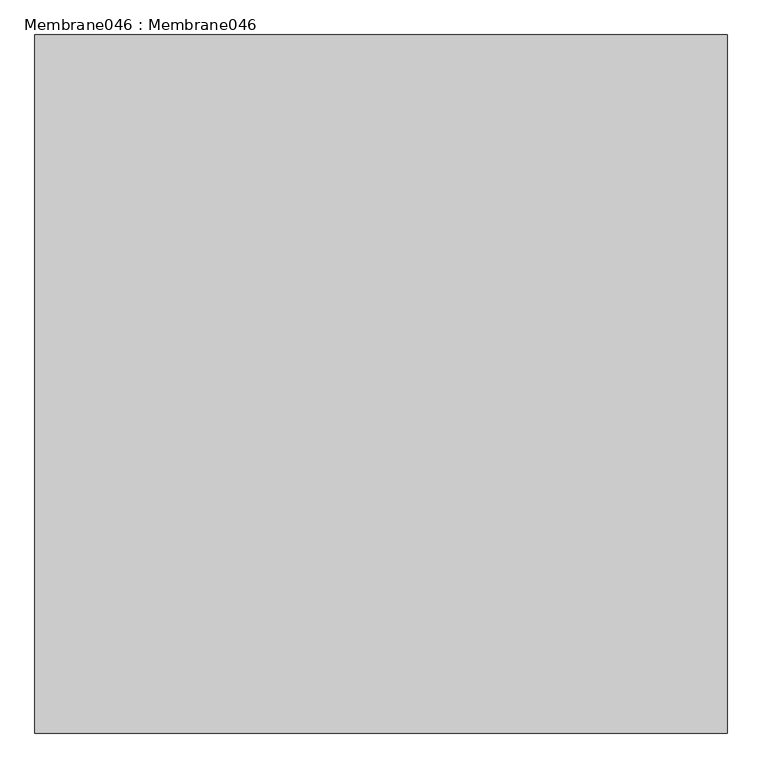
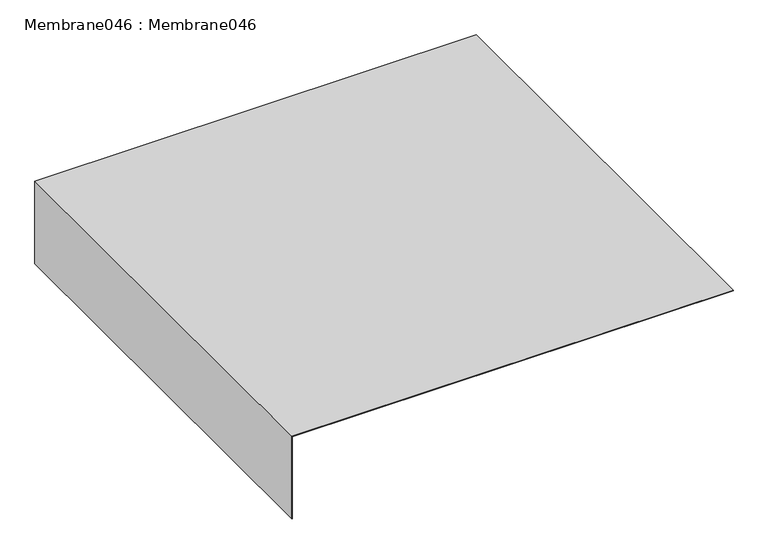
"""IFC4 building model written with IfcOpenShell, lengths in millimetres: proxy geometry, Membrane046 : Membrane046."""

from ifc_helpers import new_model, si_unit, frame, origin, place, context, project, spatial, polyline, outline, extrude, source, transform, mapped, element, save


def membrane046_membrane046_453448af(model_context):
    return source(origin(), model_context, "Body", "SweptSolid", [
        extrude(outline(polyline([(42521.46875, -475.8491821), (42521.46875, -2458.5124512), (42129.1953125, -2458.5124512), (42129.1953125, -2456.5124512), (42519.46875, -2456.5124512), (42519.46875, -475.8491821), (42521.46875, -475.8491821)])), frame((0.0, -1052.8906574, 0.0), z_axis=(0.0, 1.0, 0.0), x_axis=(0.0, 0.0, 1.0)), (0.0, 0.0, 1.0), 2000.0),
    ])


if __name__ == "__main__":
    model = new_model("IFC4")
    model_context = context("Model", 3, world=origin())
    ifc_project = project(units=[si_unit("LENGTHUNIT", "METRE", prefix="MILLI")], contexts=[model_context])
    site = spatial("IfcSite", under=ifc_project)
    building = spatial("IfcBuilding", under=site)
    placement = place(None, origin())
    membrane046_membrane046_shape = membrane046_membrane046_453448af(model_context)
    element("IfcBuildingElementProxy", 1, Name="Membrane046 : Membrane046", ObjectType="Membrane046 : Membrane046", at=placement, inside=building, context=model_context, shape_type="MappedRepresentation", body=[
        mapped(membrane046_membrane046_shape, transform((0.0, 0.0, 0.0), x_axis=(1.0, 0.0, 0.0), y_axis=(0.0, 1.0, 0.0), z_axis=(0.0, 0.0, 1.0))),
    ])
    save(model, "model.ifc")

# Revit data of these elements
# Type "Membrane046 : Membrane046"
#   NameOverride = "Membrane046"
# Element 1 (IfcBuildingElementProxy, "Membrane046 : Membrane046")
#   Materials on its faces: "2 LAYERS NO. 30 ASTM D226 ASPHALT SATURATED ORGANIC FELT"
# Materials
#   "2 LAYERS NO. 30 ASTM D226 ASPHALT SATURATED ORGANIC FELT": class "Unassigned", colour RGB 46 171 0, transparency 0
